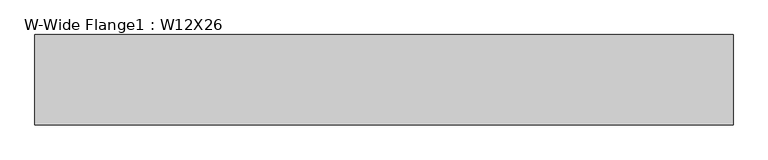
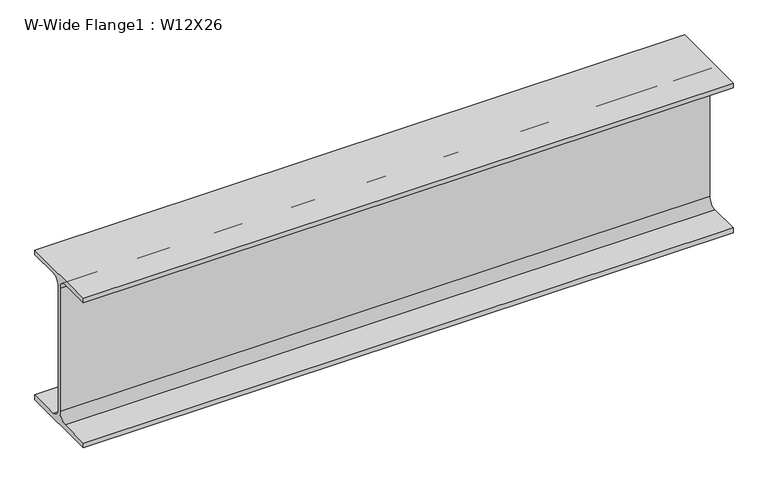
"""IFC4 building model written with IfcOpenShell, lengths in millimetres: beam geometry, W-Wide Flange1 : W12X26."""

from ifc_helpers import new_model, si_unit, point, frame, frame_2d, origin, place, context, project, spatial, polyline, circle_curve, trimmed, segment, composite_curve, outline, extrude, source, transform, mapped, element, save


def w_wide_flange1_w12x26_2e36d113(model_context):
    return source(origin(), model_context, "Body", "SweptSolid", [
        extrude(outline(composite_curve([segment(polyline([(82.423, -145.288), (82.423, -154.94), (-82.423, -154.94), (-82.423, -145.288), (-20.2565, -145.288)]), True, "CONTINUOUS"), segment(trimmed(circle_curve(frame_2d((-20.2565, -127.9525)), 17.3355), [point((-20.2565, -145.288))], [point((-2.921, -127.9525))], True, "CARTESIAN"), True, "CONTINUOUS"), segment(polyline([(-2.921, -127.9525), (-2.921, 127.9525)]), True, "CONTINUOUS"), segment(trimmed(circle_curve(frame_2d((-20.2565, 127.9525)), 17.3355), [point((-2.921, 127.9525))], [point((-20.2565, 145.288))], True, "CARTESIAN"), True, "CONTINUOUS"), segment(polyline([(-20.2565, 145.288), (-82.423, 145.288), (-82.423, 154.94), (82.423, 154.94), (82.423, 145.288), (20.2565, 145.288)]), True, "CONTINUOUS"), segment(trimmed(circle_curve(frame_2d((20.2565, 127.9525)), 17.3355), [point((20.2565, 145.288))], [point((2.921, 127.9525))], True, "CARTESIAN"), True, "CONTINUOUS"), segment(polyline([(2.921, 127.9525), (2.921, -127.9525)]), True, "CONTINUOUS"), segment(trimmed(circle_curve(frame_2d((20.2565, -127.9525)), 17.3355), [point((2.921, -127.9525))], [point((20.2565, -145.288))], True, "CARTESIAN"), True, "CONTINUOUS"), segment(polyline([(20.2565, -145.288), (82.423, -145.288)]), True, "CONTINUOUS")], self_intersect=False)), frame((-628.1482791, 0.0, 0.0), z_axis=(1.0, 0.0, 0.0), x_axis=(0.0, 1.0, 0.0)), (0.0, 0.0, 1.0), 1273.8175407),
    ])


if __name__ == "__main__":
    model = new_model("IFC4")
    model_context = context("Model", 3, world=origin())
    ifc_project = project(units=[si_unit("LENGTHUNIT", "METRE", prefix="MILLI")], contexts=[model_context])
    site = spatial("IfcSite", under=ifc_project)
    building = spatial("IfcBuilding", under=site)
    placement = place(None, origin())
    w_wide_flange1_w12x26_shape = w_wide_flange1_w12x26_2e36d113(model_context)
    element("IfcBeam", 1, ObjectType="W-Wide Flange1 : W12X26", at=placement, inside=building, context=model_context, shape_type="MappedRepresentation", body=[
        mapped(w_wide_flange1_w12x26_shape, transform((0.0, 0.0, 0.0), x_axis=(1.0, 0.0, 0.0), y_axis=(0.0, 1.0, 0.0), z_axis=(0.0, 0.0, 1.0))),
    ])
    save(model, "model.ifc")

# Revit data of these elements
# Type "W-Wide Flange1 : W12X26"
#   Assembly Code = "B10"
#   W = 26
#   Start Extension Calculation [instance default] = 10' - 0"
#   Start Extension [instance default] = -0' - 0 1/2"
#   End Extension Calculation [instance default] = 10' - 0"
#   End Extension [instance default] = -0' - 0 1/2"
#   Length [instance default] = 5' - 0"
#   bf = 0' - 6.49"
#   d = 1' - 0.2"
#   k = 0' - 1 1/16"
#   k2 = 0' - 0.6825"
#   tf = 0' - 0.38"
#   tw = 0' - 0.23"
#   A = 0.053125 SF
#   Structural Material [instance default] = Metal - Steel - ASTM A992
# Element 1 (IfcBeam, "W-Wide Flange1 : W12X26")
#   Materials on its faces: "Metal - Steel - ASTM A992"
# Materials
#   "Metal - Steel - ASTM A992": class "Metal", colour RGB 199 199 199, transparency 0
